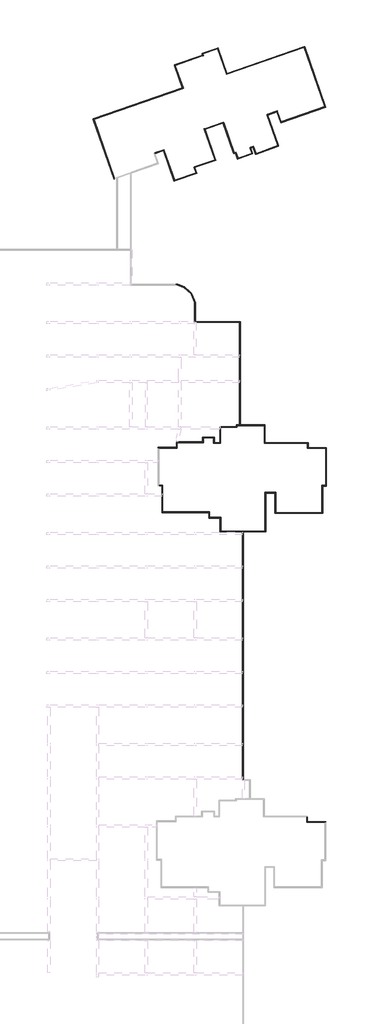
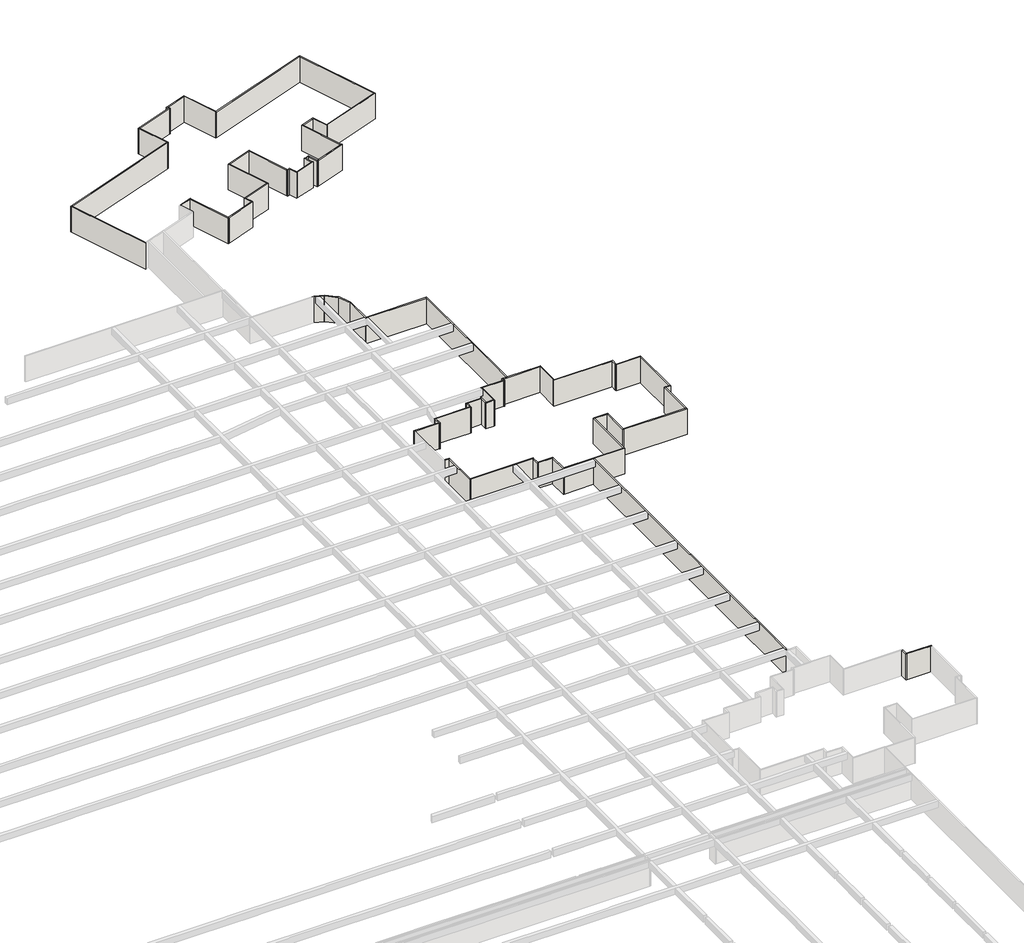
# One storey, part 6 of 14: 66 walls.
"""IFC4 building model written with IfcOpenShell, lengths in millimetres."""

from ifc_helpers import new_model, si_unit, origin, origin_with_axes, place, context, project, spatial, polyline, outline, extrude, faceted_brep, element, save

model = new_model("IFC4")

# Units and contexts
model_context = context("Model", 3, world=origin())
ifc_project = project(units=[si_unit("LENGTHUNIT", "METRE", prefix="MILLI")], contexts=[model_context])

# Site, building, storey
site = spatial("IfcSite", under=ifc_project)
building = spatial("IfcBuilding", under=site)
storey = spatial("IfcBuildingStorey", under=building, Name="户型图", Elevation=0.0)

# Walls
placement = place(None, origin())
element("IfcWall", 1, ObjectType="所有墙体", at=placement, inside=storey, context=model_context, shape_type="Brep", body=[
    faceted_brep([(-487731.9156201, -109117.5126628, 0.0), (-487731.9156201, -110017.5126628, 0.0), (-487731.9156201, -110017.5126628, 3300.0), (-487731.9156201, -109117.5126628, 3300.0), (-487611.9156201, -109117.5126628, 0.0), (-487611.9156201, -109117.5126628, 3300.0), (-487611.9156201, -109897.5126628, 3300.0), (-487611.9156201, -110017.5126628, 3300.0), (-487611.9156201, -110017.5126628, 0.0), (-487611.9156201, -109897.5126628, 0.0)], [[[0, 1, 2, 3]], [[4, 5, 6, 7, 8, 9]], [[1, 0, 4, 9, 8]], [[3, 2, 7, 6, 5]], [[0, 3, 5, 4]], [[2, 1, 8, 7]]]),
])
element("IfcWall", 2, ObjectType="所有墙体", at=placement, inside=storey, context=model_context, shape_type="Brep", body=[
    faceted_brep([(-487611.9156201, -110017.5126628, 0.0), (-484731.9156201, -110017.5126628, 0.0), (-484611.9156201, -110017.5126628, 0.0), (-484611.9156201, -110017.5126628, 3300.0), (-484731.9156201, -110017.5126628, 3300.0), (-487611.9156201, -110017.5126628, 3300.0), (-487611.9156201, -109897.5126628, 0.0), (-487611.9156201, -109897.5126628, 3300.0), (-484611.9156201, -109897.5126628, 3300.0), (-484611.9156201, -109897.5126628, 0.0)], [[[0, 1, 2, 3, 4, 5]], [[6, 7, 8, 9]], [[2, 1, 0, 6, 9]], [[5, 4, 3, 8, 7]], [[0, 5, 7, 6]], [[3, 2, 9, 8]]]),
])
element("IfcWall", 3, ObjectType="所有墙体", at=placement, inside=storey, context=model_context, shape_type="SweptSolid", body=[
    extrude(outline(polyline([(-498157.6529954, -62419.4327531), (-498157.6529954, -103033.8197785), (-498277.6529954, -103033.8197785), (-498277.6529954, -62419.4327531), (-498157.6529954, -62419.4327531)])), origin_with_axes(), (0.0, 0.0, 1.0), 3300.0),
])
element("IfcWall", 4, ObjectType="所有墙体", at=placement, inside=storey, context=model_context, shape_type="Brep", body=[
    faceted_brep([(-501839.5424455, -62419.4327531, 0.0), (-498277.6529954, -62419.4327531, 0.0), (-498157.6529954, -62419.4327531, 0.0), (-494448.2280208, -62419.4327531, 0.0), (-494448.2280208, -62419.4327531, 3300.0), (-498157.6529954, -62419.4327531, 3300.0), (-498277.6529954, -62419.4327531, 3300.0), (-501839.5424455, -62419.4327531, 3300.0), (-501839.5424455, -62299.4327531, 0.0), (-501839.5424455, -62299.4327531, 3300.0), (-494568.2280208, -62299.4327531, 3300.0), (-494448.2280208, -62299.4327531, 3300.0), (-494448.2280208, -62299.4327531, 0.0), (-494568.2280208, -62299.4327531, 0.0)], [[[0, 1, 2, 3, 4, 5, 6, 7]], [[8, 9, 10, 11, 12, 13]], [[3, 2, 1, 0, 8, 13, 12]], [[7, 6, 5, 4, 11, 10, 9]], [[4, 3, 12, 11]], [[0, 7, 9, 8]]]),
])
element("IfcWall", 5, ObjectType="所有墙体", at=placement, inside=storey, context=model_context, shape_type="Brep", body=[
    faceted_brep([(-494448.2280208, -62299.4327531, 0.0), (-494448.2280208, -56065.482039, 0.0), (-494448.2280208, -55945.482039, 0.0), (-494448.2280208, -55945.482039, 3300.0), (-494448.2280208, -56065.482039, 3300.0), (-494448.2280208, -62299.4327531, 3300.0), (-494568.2280208, -62299.4327531, 0.0), (-494568.2280208, -62299.4327531, 3300.0), (-494568.2280208, -55945.482039, 3300.0), (-494568.2280208, -55945.482039, 0.0)], [[[0, 1, 2, 3, 4, 5]], [[6, 7, 8, 9]], [[2, 1, 0, 6, 9]], [[5, 4, 3, 8, 7]], [[0, 5, 7, 6]], [[3, 2, 9, 8]]]),
])
element("IfcWall", 6, ObjectType="所有墙体", at=placement, inside=storey, context=model_context, shape_type="Brep", body=[
    faceted_brep([(-494448.2280208, -56065.482039, 0.0), (-492943.6459925, -56065.482039, 0.0), (-492823.6459925, -56065.482039, 0.0), (-492823.6459925, -56065.482039, 3300.0), (-492943.6459925, -56065.482039, 3300.0), (-494448.2280208, -56065.482039, 3300.0), (-494448.2280208, -55945.482039, 0.0), (-494448.2280208, -55945.482039, 3300.0), (-492823.6459925, -55945.482039, 3300.0), (-492823.6459925, -55945.482039, 0.0)], [[[0, 1, 2, 3, 4, 5]], [[6, 7, 8, 9]], [[2, 1, 0, 6, 9]], [[5, 4, 3, 8, 7]], [[0, 5, 7, 6]], [[3, 2, 9, 8]]]),
])
element("IfcWall", 7, ObjectType="所有墙体", at=placement, inside=storey, context=model_context, shape_type="Brep", body=[
    faceted_brep([(-492943.6459925, -56065.482039, 0.0), (-492943.6459925, -59371.7887885, 0.0), (-492943.6459925, -59371.7887885, 3300.0), (-492943.6459925, -56065.482039, 3300.0), (-492823.6459925, -56065.482039, 0.0), (-492823.6459925, -56065.482039, 3300.0), (-492823.6459925, -59251.7887885, 3300.0), (-492823.6459925, -59371.7887885, 3300.0), (-492823.6459925, -59371.7887885, 0.0), (-492823.6459925, -59251.7887885, 0.0)], [[[0, 1, 2, 3]], [[4, 5, 6, 7, 8, 9]], [[1, 0, 4, 9, 8]], [[3, 2, 7, 6, 5]], [[0, 3, 5, 4]], [[2, 1, 8, 7]]]),
])
element("IfcWall", 8, ObjectType="所有墙体", at=placement, inside=storey, context=model_context, shape_type="Brep", body=[
    faceted_brep([(-492823.6459925, -59371.7887885, 0.0), (-485136.3735207, -59371.7887885, 0.0), (-485136.3735207, -59371.7887885, 3300.0), (-492823.6459925, -59371.7887885, 3300.0), (-492823.6459925, -59251.7887885, 0.0), (-492823.6459925, -59251.7887885, 3300.0), (-485256.3735207, -59251.7887885, 3300.0), (-485136.3735207, -59251.7887885, 3300.0), (-485136.3735207, -59251.7887885, 0.0), (-485256.3735207, -59251.7887885, 0.0)], [[[0, 1, 2, 3]], [[4, 5, 6, 7, 8, 9]], [[1, 0, 4, 9, 8]], [[3, 2, 7, 6, 5]], [[0, 3, 5, 4]], [[2, 1, 8, 7]]]),
])
element("IfcWall", 9, ObjectType="所有墙体", at=placement, inside=storey, context=model_context, shape_type="Brep", body=[
    faceted_brep([(-485136.3735207, -59251.7887885, 0.0), (-485136.3735207, -54901.4809263, 0.0), (-485136.3735207, -54781.4809263, 0.0), (-485136.3735207, -54781.4809263, 3300.0), (-485136.3735207, -54901.4809263, 3300.0), (-485136.3735207, -59251.7887885, 3300.0), (-485256.3735207, -59251.7887885, 0.0), (-485256.3735207, -59251.7887885, 3300.0), (-485256.3735207, -54781.4809263, 3300.0), (-485256.3735207, -54781.4809263, 0.0)], [[[0, 1, 2, 3, 4, 5]], [[6, 7, 8, 9]], [[2, 1, 0, 6, 9]], [[5, 4, 3, 8, 7]], [[0, 5, 7, 6]], [[3, 2, 9, 8]]]),
])
element("IfcWall", 10, ObjectType="所有墙体", at=placement, inside=storey, context=model_context, shape_type="Brep", body=[
    faceted_brep([(-485136.3735207, -54901.4809263, 0.0), (-484519.0828774, -54901.4809263, 0.0), (-484519.0828774, -54901.4809263, 3300.0), (-485136.3735207, -54901.4809263, 3300.0), (-485136.3735207, -54781.4809263, 0.0), (-485136.3735207, -54781.4809263, 3300.0), (-484639.0828774, -54781.4809263, 3300.0), (-484519.0828774, -54781.4809263, 3300.0), (-484519.0828774, -54781.4809263, 0.0), (-484639.0828774, -54781.4809263, 0.0)], [[[0, 1, 2, 3]], [[4, 5, 6, 7, 8, 9]], [[1, 0, 4, 9, 8]], [[3, 2, 7, 6, 5]], [[0, 3, 5, 4]], [[2, 1, 8, 7]]]),
])
element("IfcWall", 11, ObjectType="所有墙体", at=placement, inside=storey, context=model_context, shape_type="Brep", body=[
    faceted_brep([(-484519.0828774, -54781.4809263, 0.0), (-484519.0828774, -48583.8215635, 0.0), (-484519.0828774, -48583.8215635, 3300.0), (-484519.0828774, -54781.4809263, 3300.0), (-484639.0828774, -54781.4809263, 0.0), (-484639.0828774, -54781.4809263, 3300.0), (-484639.0828774, -48703.8215635, 3300.0), (-484639.0828774, -48583.8215635, 3300.0), (-484639.0828774, -48583.8215635, 0.0), (-484639.0828774, -48703.8215635, 0.0)], [[[0, 1, 2, 3]], [[4, 5, 6, 7, 8, 9]], [[1, 0, 4, 9, 8]], [[3, 2, 7, 6, 5]], [[0, 3, 5, 4]], [[2, 1, 8, 7]]]),
])
element("IfcWall", 12, ObjectType="所有墙体", at=placement, inside=storey, context=model_context, shape_type="Brep", body=[
    faceted_brep([(-484639.0828774, -48583.8215635, 0.0), (-487495.1396851, -48583.8215635, 0.0), (-487615.1396851, -48583.8215635, 0.0), (-487615.1396851, -48583.8215635, 3300.0), (-487495.1396851, -48583.8215635, 3300.0), (-484639.0828774, -48583.8215635, 3300.0), (-484639.0828774, -48703.8215635, 0.0), (-484639.0828774, -48703.8215635, 3300.0), (-487615.1396851, -48703.8215635, 3300.0), (-487615.1396851, -48703.8215635, 0.0)], [[[0, 1, 2, 3, 4, 5]], [[6, 7, 8, 9]], [[2, 1, 0, 6, 9]], [[5, 4, 3, 8, 7]], [[0, 5, 7, 6]], [[3, 2, 9, 8]]]),
])
element("IfcWall", 13, ObjectType="所有墙体", at=placement, inside=storey, context=model_context, shape_type="Brep", body=[
    faceted_brep([(-487495.1396851, -48583.8215635, 0.0), (-487495.1396851, -47772.3075196, 0.0), (-487495.1396851, -47772.3075196, 3300.0), (-487495.1396851, -48583.8215635, 3300.0), (-487615.1396851, -48583.8215635, 0.0), (-487615.1396851, -48583.8215635, 3300.0), (-487615.1396851, -47892.3075196, 3300.0), (-487615.1396851, -47772.3075196, 3300.0), (-487615.1396851, -47772.3075196, 0.0), (-487615.1396851, -47892.3075196, 0.0)], [[[0, 1, 2, 3]], [[4, 5, 6, 7, 8, 9]], [[1, 0, 4, 9, 8]], [[3, 2, 7, 6, 5]], [[0, 3, 5, 4]], [[2, 1, 8, 7]]]),
])
element("IfcWall", 14, ObjectType="所有墙体", at=placement, inside=storey, context=model_context, shape_type="Brep", body=[
    faceted_brep([(-487615.1396851, -47772.3075196, 0.0), (-494595.1396851, -47772.3075196, 0.0), (-494715.1396851, -47772.3075196, 0.0), (-494715.1396851, -47772.3075196, 3300.0), (-494595.1396851, -47772.3075196, 3300.0), (-487615.1396851, -47772.3075196, 3300.0), (-487615.1396851, -47892.3075196, 0.0), (-487615.1396851, -47892.3075196, 3300.0), (-494715.1396851, -47892.3075196, 3300.0), (-494715.1396851, -47892.3075196, 0.0)], [[[0, 1, 2, 3, 4, 5]], [[6, 7, 8, 9]], [[2, 1, 0, 6, 9]], [[5, 4, 3, 8, 7]], [[0, 5, 7, 6]], [[3, 2, 9, 8]]]),
])
element("IfcWall", 15, ObjectType="所有墙体", at=placement, inside=storey, context=model_context, shape_type="Brep", body=[
    faceted_brep([(-494595.1396851, -47772.3075196, 0.0), (-494595.1396851, -44872.3075196, 0.0), (-494595.1396851, -44872.3075196, 3300.0), (-494595.1396851, -47772.3075196, 3300.0), (-494715.1396851, -47772.3075196, 0.0), (-494715.1396851, -47772.3075196, 3300.0), (-494715.1396851, -44992.3075196, 3300.0), (-494715.1396851, -44872.3075196, 3300.0), (-494715.1396851, -44872.3075196, 0.0), (-494715.1396851, -44992.3075196, 0.0)], [[[0, 1, 2, 3]], [[4, 5, 6, 7, 8, 9]], [[1, 0, 4, 9, 8]], [[3, 2, 7, 6, 5]], [[0, 3, 5, 4]], [[2, 1, 8, 7]]]),
])
element("IfcWall", 16, ObjectType="所有墙体", at=placement, inside=storey, context=model_context, shape_type="Brep", body=[
    faceted_brep([(-494715.1396851, -44872.3075196, 0.0), (-498635.1396851, -44872.3075196, 0.0), (-498755.1396851, -44872.3075196, 0.0), (-499195.1396851, -44872.3075196, 0.0), (-499195.1396851, -44872.3075196, 3300.0), (-498755.1396851, -44872.3075196, 3300.0), (-498635.1396851, -44872.3075196, 3300.0), (-494715.1396851, -44872.3075196, 3300.0), (-494715.1396851, -44992.3075196, 0.0), (-494715.1396851, -44992.3075196, 3300.0), (-499195.1396851, -44992.3075196, 3300.0), (-499195.1396851, -44992.3075196, 0.0)], [[[0, 1, 2, 3, 4, 5, 6, 7]], [[8, 9, 10, 11]], [[3, 2, 1, 0, 8, 11]], [[7, 6, 5, 4, 10, 9]], [[0, 7, 9, 8]], [[4, 3, 11, 10]]]),
])
element("IfcWall", 17, ObjectType="所有墙体", at=placement, inside=storey, context=model_context, shape_type="Brep", body=[
    faceted_brep([(-499315.1396851, -44872.3075196, 0.0), (-499315.1396851, -45172.3075196, 0.0), (-499315.1396851, -45292.3075196, 0.0), (-499315.1396851, -45292.3075196, 3300.0), (-499315.1396851, -45172.3075196, 3300.0), (-499315.1396851, -44872.3075196, 3300.0), (-499195.1396851, -44872.3075196, 0.0), (-499195.1396851, -44872.3075196, 3300.0), (-499195.1396851, -44992.3075196, 3300.0), (-499195.1396851, -45292.3075196, 3300.0), (-499195.1396851, -45292.3075196, 0.0), (-499195.1396851, -44992.3075196, 0.0)], [[[0, 1, 2, 3, 4, 5]], [[6, 7, 8, 9, 10, 11]], [[2, 1, 0, 6, 11, 10]], [[5, 4, 3, 9, 8, 7]], [[0, 5, 7, 6]], [[3, 2, 10, 9]]]),
])
element("IfcWall", 18, ObjectType="所有墙体", at=placement, inside=storey, context=model_context, shape_type="Brep", body=[
    faceted_brep([(-499315.1396851, -45172.3075196, 0.0), (-502015.1396851, -45172.3075196, 0.0), (-502015.1396851, -45172.3075196, 2500.0), (-502015.1396851, -45172.3075196, 3300.0), (-501895.1396851, -45172.3075196, 3300.0), (-499315.1396851, -45172.3075196, 3300.0), (-499315.1396851, -45292.3075196, 0.0), (-499315.1396851, -45292.3075196, 3300.0), (-501895.1396851, -45292.3075196, 3300.0), (-502015.1396851, -45292.3075196, 3300.0), (-502015.1396851, -45292.3075196, 0.0), (-501895.1396851, -45292.3075196, 0.0)], [[[0, 1, 2, 3, 4, 5]], [[6, 7, 8, 9, 10, 11]], [[1, 0, 6, 11, 10]], [[5, 4, 3, 9, 8, 7]], [[0, 5, 7, 6]], [[3, 2, 1, 10, 9]]]),
])
element("IfcWall", 19, ObjectType="所有墙体", at=placement, inside=storey, context=model_context, shape_type="Brep", body=[
    faceted_brep([(-502015.1396851, -45292.3075196, 0.0), (-502015.1396851, -47772.3075196, 0.0), (-502015.1396851, -47892.3075196, 0.0), (-502015.1396851, -47892.3075196, 3300.0), (-502015.1396851, -47772.3075196, 3300.0), (-502015.1396851, -45292.3075196, 3300.0), (-501895.1396851, -45292.3075196, 0.0), (-501895.1396851, -45292.3075196, 3300.0), (-501895.1396851, -47892.3075196, 3300.0), (-501895.1396851, -47892.3075196, 0.0)], [[[0, 1, 2, 3, 4, 5]], [[6, 7, 8, 9]], [[2, 1, 0, 6, 9]], [[5, 4, 3, 8, 7]], [[0, 5, 7, 6]], [[3, 2, 9, 8]]]),
])
element("IfcWall", 20, ObjectType="所有墙体", at=placement, inside=storey, context=model_context, shape_type="Brep", body=[
    faceted_brep([(-502015.1396851, -47772.3075196, 0.0), (-502895.1396851, -47772.3075196, 0.0), (-503015.1396851, -47772.3075196, 0.0), (-503015.1396851, -47772.3075196, 3300.0), (-502895.1396851, -47772.3075196, 3300.0), (-502015.1396851, -47772.3075196, 3300.0), (-502015.1396851, -47892.3075196, 0.0), (-502015.1396851, -47892.3075196, 3300.0), (-503015.1396851, -47892.3075196, 3300.0), (-503015.1396851, -47892.3075196, 0.0)], [[[0, 1, 2, 3, 4, 5]], [[6, 7, 8, 9]], [[2, 1, 0, 6, 9]], [[5, 4, 3, 8, 7]], [[0, 5, 7, 6]], [[3, 2, 9, 8]]]),
])
element("IfcWall", 21, ObjectType="所有墙体", at=placement, inside=storey, context=model_context, shape_type="Brep", body=[
    faceted_brep([(-502895.1396851, -47772.3075196, 0.0), (-502895.1396851, -46872.3075196, 0.0), (-502895.1396851, -46872.3075196, 3300.0), (-502895.1396851, -47772.3075196, 3300.0), (-503015.1396851, -47772.3075196, 0.0), (-503015.1396851, -47772.3075196, 3300.0), (-503015.1396851, -46992.3075196, 3300.0), (-503015.1396851, -46872.3075196, 3300.0), (-503015.1396851, -46872.3075196, 0.0), (-503015.1396851, -46992.3075196, 0.0)], [[[0, 1, 2, 3]], [[4, 5, 6, 7, 8, 9]], [[1, 0, 4, 9, 8]], [[3, 2, 7, 6, 5]], [[0, 3, 5, 4]], [[2, 1, 8, 7]]]),
])
element("IfcWall", 22, ObjectType="所有墙体", at=placement, inside=storey, context=model_context, shape_type="Brep", body=[
    faceted_brep([(-503015.1396851, -46872.3075196, 0.0), (-504815.1396851, -46872.3075196, 0.0), (-504815.1396851, -46872.3075196, 3300.0), (-503015.1396851, -46872.3075196, 3300.0), (-503015.1396851, -46992.3075196, 0.0), (-503015.1396851, -46992.3075196, 3300.0), (-504695.1396851, -46992.3075196, 3300.0), (-504815.1396851, -46992.3075196, 3300.0), (-504815.1396851, -46992.3075196, 0.0), (-504695.1396851, -46992.3075196, 0.0)], [[[0, 1, 2, 3]], [[4, 5, 6, 7, 8, 9]], [[1, 0, 4, 9, 8]], [[3, 2, 7, 6, 5]], [[0, 3, 5, 4]], [[2, 1, 8, 7]]]),
])
element("IfcWall", 23, ObjectType="所有墙体", at=placement, inside=storey, context=model_context, shape_type="Brep", body=[
    faceted_brep([(-504815.1396851, -46992.3075196, 0.0), (-504815.1396851, -47655.7967618, 0.0), (-504815.1396851, -47775.7967618, 0.0), (-504815.1396851, -47775.7967618, 3300.0), (-504815.1396851, -47655.7967618, 3300.0), (-504815.1396851, -46992.3075196, 3300.0), (-504695.1396851, -46992.3075196, 0.0), (-504695.1396851, -46992.3075196, 3300.0), (-504695.1396851, -47775.7967618, 3300.0), (-504695.1396851, -47775.7967618, 0.0)], [[[0, 1, 2, 3, 4, 5]], [[6, 7, 8, 9]], [[2, 1, 0, 6, 9]], [[5, 4, 3, 8, 7]], [[0, 5, 7, 6]], [[3, 2, 9, 8]]]),
])
element("IfcWall", 24, ObjectType="所有墙体", at=placement, inside=storey, context=model_context, shape_type="Brep", body=[
    faceted_brep([(-504815.1396851, -47655.7967618, 0.0), (-509115.1396851, -47655.7967618, 0.0), (-509115.1396851, -47655.7967618, 3300.0), (-504815.1396851, -47655.7967618, 3300.0), (-504815.1396851, -47775.7967618, 0.0), (-504815.1396851, -47775.7967618, 3300.0), (-508995.1396851, -47775.7967618, 3300.0), (-509115.1396851, -47775.7967618, 3300.0), (-509115.1396851, -47775.7967618, 0.0), (-508995.1396851, -47775.7967618, 0.0)], [[[0, 1, 2, 3]], [[4, 5, 6, 7, 8, 9]], [[1, 0, 4, 9, 8]], [[3, 2, 7, 6, 5]], [[0, 3, 5, 4]], [[2, 1, 8, 7]]]),
])
element("IfcWall", 25, ObjectType="所有墙体", at=placement, inside=storey, context=model_context, shape_type="Brep", body=[
    faceted_brep([(-509115.1396851, -47775.7967618, 0.0), (-509115.1396851, -48542.2511208, 0.0), (-509115.1396851, -48662.2511208, 0.0), (-509115.1396851, -48662.2511208, 3300.0), (-509115.1396851, -48542.2511208, 3300.0), (-509115.1396851, -47775.7967618, 3300.0), (-508995.1396851, -47775.7967618, 0.0), (-508995.1396851, -47775.7967618, 3300.0), (-508995.1396851, -48662.2511208, 3300.0), (-508995.1396851, -48662.2511208, 0.0)], [[[0, 1, 2, 3, 4, 5]], [[6, 7, 8, 9]], [[2, 1, 0, 6, 9]], [[5, 4, 3, 8, 7]], [[0, 5, 7, 6]], [[3, 2, 9, 8]]]),
])
element("IfcWall", 26, ObjectType="所有墙体", at=placement, inside=storey, context=model_context, shape_type="Brep", body=[
    faceted_brep([(-509115.1396851, -48542.2511208, 0.0), (-512115.1621146, -48542.2511208, 0.0), (-512115.1621146, -48542.2511208, 3300.0), (-509115.1396851, -48542.2511208, 3300.0), (-509115.1396851, -48662.2511208, 0.0), (-509115.1396851, -48662.2511208, 3300.0), (-511995.1621146, -48662.2511208, 3300.0), (-512115.1621146, -48662.2511208, 3300.0), (-512115.1621146, -48662.2511208, 0.0), (-511995.1621146, -48662.2511208, 0.0)], [[[0, 1, 2, 3]], [[4, 5, 6, 7, 8, 9]], [[1, 0, 4, 9, 8]], [[3, 2, 7, 6, 5]], [[0, 3, 5, 4]], [[2, 1, 8, 7]]]),
])
element("IfcWall", 27, ObjectType="所有墙体", at=placement, inside=storey, context=model_context, shape_type="Brep", body=[
    faceted_brep([(-511995.1621146, -54862.2511208, 0.0), (-511515.1621146, -54862.2511208, 0.0), (-511395.1621146, -54862.2511208, 0.0), (-511395.1621146, -54862.2511208, 3300.0), (-511515.1621146, -54862.2511208, 3300.0), (-511995.1621146, -54862.2511208, 3300.0), (-511995.1621146, -54742.2511208, 0.0), (-511995.1621146, -54742.2511208, 3300.0), (-511395.1621146, -54742.2511208, 3300.0), (-511395.1621146, -54742.2511208, 0.0)], [[[0, 1, 2, 3, 4, 5]], [[6, 7, 8, 9]], [[2, 1, 0, 6, 9]], [[5, 4, 3, 8, 7]], [[0, 5, 7, 6]], [[3, 2, 9, 8]]]),
])
element("IfcWall", 28, ObjectType="所有墙体", at=placement, inside=storey, context=model_context, shape_type="Brep", body=[
    faceted_brep([(-511515.1621146, -54862.2511208, 0.0), (-511515.1621146, -59259.003002, 0.0), (-511515.1621146, -59259.003002, 3300.0), (-511515.1621146, -54862.2511208, 3300.0), (-511395.1621146, -54862.2511208, 0.0), (-511395.1621146, -54862.2511208, 3300.0), (-511395.1621146, -59139.003002, 3300.0), (-511395.1621146, -59259.003002, 3300.0), (-511395.1621146, -59259.003002, 0.0), (-511395.1621146, -59139.003002, 0.0)], [[[0, 1, 2, 3]], [[4, 5, 6, 7, 8, 9]], [[1, 0, 4, 9, 8]], [[3, 2, 7, 6, 5]], [[0, 3, 5, 4]], [[2, 1, 8, 7]]]),
])
element("IfcWall", 29, ObjectType="所有墙体", at=placement, inside=storey, context=model_context, shape_type="Brep", body=[
    faceted_brep([(-511395.1621146, -59259.003002, 0.0), (-503815.1621146, -59259.003002, 0.0), (-503695.1621146, -59259.003002, 0.0), (-503695.1621146, -59259.003002, 3300.0), (-503815.1621146, -59259.003002, 3300.0), (-511395.1621146, -59259.003002, 3300.0), (-511395.1621146, -59139.003002, 0.0), (-511395.1621146, -59139.003002, 3300.0), (-503695.1621146, -59139.003002, 3300.0), (-503695.1621146, -59139.003002, 0.0)], [[[0, 1, 2, 3, 4, 5]], [[6, 7, 8, 9]], [[2, 1, 0, 6, 9]], [[5, 4, 3, 8, 7]], [[0, 5, 7, 6]], [[3, 2, 9, 8]]]),
])
element("IfcWall", 30, ObjectType="所有墙体", at=placement, inside=storey, context=model_context, shape_type="Brep", body=[
    faceted_brep([(-503815.1621146, -59259.003002, 0.0), (-503815.1621146, -60159.003002, 0.0), (-503815.1621146, -60159.003002, 3300.0), (-503815.1621146, -59259.003002, 3300.0), (-503695.1621146, -59259.003002, 0.0), (-503695.1621146, -59259.003002, 3300.0), (-503695.1621146, -60039.003002, 3300.0), (-503695.1621146, -60159.003002, 3300.0), (-503695.1621146, -60159.003002, 0.0), (-503695.1621146, -60039.003002, 0.0)], [[[0, 1, 2, 3]], [[4, 5, 6, 7, 8, 9]], [[1, 0, 4, 9, 8]], [[3, 2, 7, 6, 5]], [[0, 3, 5, 4]], [[2, 1, 8, 7]]]),
])
element("IfcWall", 31, ObjectType="所有墙体", at=placement, inside=storey, context=model_context, shape_type="Brep", body=[
    faceted_brep([(-503695.1621146, -60159.003002, 0.0), (-501959.5424455, -60159.003002, 0.0), (-501839.5424455, -60159.003002, 0.0), (-501839.5424455, -60159.003002, 3300.0), (-501959.5424455, -60159.003002, 3300.0), (-503695.1621146, -60159.003002, 3300.0), (-503695.1621146, -60039.003002, 0.0), (-503695.1621146, -60039.003002, 3300.0), (-501839.5424455, -60039.003002, 3300.0), (-501839.5424455, -60039.003002, 0.0)], [[[0, 1, 2, 3, 4, 5]], [[6, 7, 8, 9]], [[2, 1, 0, 6, 9]], [[5, 4, 3, 8, 7]], [[0, 5, 7, 6]], [[3, 2, 9, 8]]]),
])
element("IfcWall", 32, ObjectType="所有墙体", at=placement, inside=storey, context=model_context, shape_type="Brep", body=[
    faceted_brep([(-501959.5424455, -60159.003002, 0.0), (-501959.5424455, -62419.4327531, 0.0), (-501959.5424455, -62419.4327531, 3300.0), (-501959.5424455, -60159.003002, 3300.0), (-501839.5424455, -60159.003002, 0.0), (-501839.5424455, -60159.003002, 3300.0), (-501839.5424455, -62299.4327531, 3300.0), (-501839.5424455, -62419.4327531, 3300.0), (-501839.5424455, -62419.4327531, 0.0), (-501839.5424455, -62299.4327531, 0.0)], [[[0, 1, 2, 3]], [[4, 5, 6, 7, 8, 9]], [[1, 0, 4, 9, 8]], [[3, 2, 7, 6, 5]], [[0, 3, 5, 4]], [[2, 1, 8, 7]]]),
])
element("IfcWall", 33, ObjectType="所有墙体", at=placement, inside=storey, context=model_context, shape_type="Brep", body=[
    faceted_brep([(-498635.1396851, -44872.3075196, 0.0), (-498635.1396851, -27939.4327531, 0.0), (-498635.1396851, -27939.4327531, 3300.0), (-498635.1396851, -44872.3075196, 3300.0), (-498755.1396851, -44872.3075196, 0.0), (-498755.1396851, -44872.3075196, 3300.0), (-498755.1396851, -28059.4327531, 3300.0), (-498755.1396851, -27939.4327531, 3300.0), (-498755.1396851, -27939.4327531, 0.0), (-498755.1396851, -28059.4327531, 0.0)], [[[0, 1, 2, 3]], [[4, 5, 6, 7, 8, 9]], [[1, 0, 4, 9, 8]], [[3, 2, 7, 6, 5]], [[0, 3, 5, 4]], [[2, 1, 8, 7]]]),
])
element("IfcWall", 34, ObjectType="所有墙体", at=placement, inside=storey, context=model_context, shape_type="Brep", body=[
    faceted_brep([(-498755.1396851, -27939.4327531, 0.0), (-506035.1396851, -27939.4327531, 0.0), (-506155.1396851, -27939.4327531, 0.0), (-506155.1396851, -27939.4327531, 3300.0), (-506035.1396851, -27939.4327531, 3300.0), (-498755.1396851, -27939.4327531, 3300.0), (-498755.1396851, -28059.4327531, 0.0), (-498755.1396851, -28059.4327531, 3300.0), (-506067.6529954, -28059.4327531, 3300.0), (-506155.1396851, -28059.4327531, 3300.0), (-506155.1396851, -28059.4327531, 2500.0), (-506155.1396851, -28059.4327531, 0.0)], [[[0, 1, 2, 3, 4, 5]], [[6, 7, 8, 9, 10, 11]], [[2, 1, 0, 6, 11]], [[5, 4, 3, 9, 8, 7]], [[0, 5, 7, 6]], [[3, 2, 11, 10, 9]]]),
])
element("IfcWall", 35, ObjectType="所有墙体", at=placement, inside=storey, context=model_context, shape_type="Brep", body=[
    faceted_brep([(-506035.1396851, -27939.4327531, 0.0), (-506035.1396851, -24747.7021405, 0.0), (-506035.1396851, -24747.7021405, 3300.0), (-506035.1396851, -27939.4327531, 3300.0), (-506155.1396851, -27939.4327531, 0.0), (-506155.1396851, -27939.4327531, 3300.0), (-506155.1396851, -27859.4327531, 3300.0), (-506155.1396851, -24771.1633658, 3300.0), (-506155.1396851, -24452.5434105, 3300.0), (-506155.1396851, -24452.5434105, 0.0), (-506155.1396851, -24771.1633658, 0.0)], [[[0, 1, 2, 3]], [[4, 5, 6, 7, 8, 9, 10]], [[1, 0, 4, 10, 9]], [[3, 2, 8, 7, 6, 5]], [[0, 3, 5, 4]], [[2, 1, 9, 8]]]),
])
element("IfcWall", 36, ObjectType="所有墙体", at=placement, inside=storey, context=model_context, shape_type="Brep", body=[
    faceted_brep([(-506155.1396851, -24452.5434105, 0.0), (-506634.5565644, -23273.3427667, 0.0), (-506634.5565644, -23273.3427667, 3300.0), (-506155.1396851, -24452.5434105, 3300.0), (-506155.1396851, -24771.1633658, 0.0), (-506155.1396851, -24771.1633658, 3300.0), (-506734.7494264, -23345.5227396, 3300.0), (-506833.3243097, -23103.0624283, 3300.0), (-506833.3243097, -23103.0624283, 0.0), (-506734.7494264, -23345.5227396, 0.0)], [[[0, 1, 2, 3]], [[4, 5, 6, 7, 8, 9]], [[1, 0, 4, 9, 8]], [[3, 2, 7, 6, 5]], [[0, 3, 5, 4]], [[2, 1, 8, 7]]]),
])
element("IfcWall", 37, ObjectType="所有墙体", at=placement, inside=storey, context=model_context, shape_type="SweptSolid", body=[
    extrude(outline(polyline([(-507820.7587047, -22257.147198), (-506833.3243097, -23103.0624283), (-506734.7494264, -23345.5227396), (-507883.1414859, -22361.7183083), (-507820.7587047, -22257.147198)])), origin_with_axes(), (0.0, 0.0, 1.0), 3300.0),
])
element("IfcWall", 38, ObjectType="所有墙体", at=placement, inside=storey, context=model_context, shape_type="Brep", body=[
    faceted_brep([(-507820.7587047, -22257.147198, 0.0), (-508906.5049791, -21839.2569935, 0.0), (-508906.5049791, -21839.2569935, 3300.0), (-507820.7587047, -22257.147198, 3300.0), (-507883.1414859, -22361.7183083, 0.0), (-507883.1414859, -22361.7183083, 3300.0), (-508928.8010117, -21959.2569935, 3300.0), (-509240.5804015, -21839.2569935, 3300.0), (-509240.5804015, -21839.2569935, 0.0), (-508928.8010117, -21959.2569935, 0.0)], [[[0, 1, 2, 3]], [[4, 5, 6, 7, 8, 9]], [[1, 0, 4, 9, 8]], [[3, 2, 7, 6, 5]], [[0, 3, 5, 4]], [[2, 1, 8, 7]]]),
])
element("IfcWall", 39, ObjectType="所有墙体", at=placement, inside=storey, context=model_context, shape_type="Brep", body=[
    faceted_brep([(-512675.4931907, -384.9532556, 0.0), (-511246.2354826, 111.3129454, 0.0), (-511132.8745486, 150.6740766, 0.0), (-511132.8745486, 150.6740766, 3300.0), (-511246.2354826, 111.3129454, 3300.0), (-512675.4931907, -384.9532556, 3300.0), (-512714.8543218, -271.5923217, 0.0), (-512714.8543218, -271.5923217, 3300.0), (-511172.2356797, 264.0350106, 3300.0), (-511172.2356797, 264.0350106, 0.0)], [[[0, 1, 2, 3, 4, 5]], [[6, 7, 8, 9]], [[2, 1, 0, 6, 9]], [[5, 4, 3, 8, 7]], [[0, 5, 7, 6]], [[3, 2, 9, 8]]]),
])
element("IfcWall", 40, ObjectType="所有墙体", at=placement, inside=storey, context=model_context, shape_type="Brep", body=[
    faceted_brep([(-511246.2354826, 111.3129454, 0.0), (-509502.0327403, -4912.0297855, 0.0), (-509502.0327403, -4912.0297855, 3300.0), (-511246.2354826, 111.3129454, 3300.0), (-511132.8745486, 150.6740766, 0.0), (-511132.8745486, 150.6740766, 3300.0), (-509428.0329375, -4759.3077204, 3300.0), (-509388.6718063, -4872.6686544, 3300.0), (-509388.6718063, -4872.6686544, 0.0), (-509428.0329375, -4759.3077204, 0.0)], [[[0, 1, 2, 3]], [[4, 5, 6, 7, 8, 9]], [[1, 0, 4, 9, 8]], [[3, 2, 7, 6, 5]], [[0, 3, 5, 4]], [[2, 1, 8, 7]]]),
])
element("IfcWall", 41, ObjectType="所有墙体", at=placement, inside=storey, context=model_context, shape_type="Brep", body=[
    faceted_brep([(-509388.6718063, -4872.6686544, 0.0), (-505756.5673718, -3611.5310307, 0.0), (-505756.5673718, -3611.5310307, 3300.0), (-509388.6718063, -4872.6686544, 3300.0), (-509428.0329375, -4759.3077204, 0.0), (-509428.0329375, -4759.3077204, 3300.0), (-505910.7131052, -3538.0255532, 3300.0), (-505797.3433424, -3498.6613566, 3300.0), (-505797.3433424, -3498.6613566, 0.0), (-505910.7131052, -3538.0255532, 0.0)], [[[0, 1, 2, 3]], [[4, 5, 6, 7, 8, 9]], [[1, 0, 4, 9, 8]], [[3, 2, 7, 6, 5]], [[0, 3, 5, 4]], [[2, 1, 8, 7]]]),
])
element("IfcWall", 42, ObjectType="所有墙体", at=placement, inside=storey, context=model_context, shape_type="Brep", body=[
    faceted_brep([(-505797.3433424, -3498.6613566, 0.0), (-506096.3406643, -2671.0236624, 0.0), (-506137.1166349, -2558.1539883, 0.0), (-506137.1166349, -2558.1539883, 3300.0), (-506096.3406643, -2671.0236624, 3300.0), (-505797.3433424, -3498.6613566, 3300.0), (-505910.7131052, -3538.0255532, 0.0), (-505910.7131052, -3538.0255532, 3300.0), (-506250.4863977, -2597.518185, 3300.0), (-506250.4863977, -2597.518185, 0.0)], [[[0, 1, 2, 3, 4, 5]], [[6, 7, 8, 9]], [[2, 1, 0, 6, 9]], [[5, 4, 3, 8, 7]], [[0, 5, 7, 6]], [[3, 2, 9, 8]]]),
])
element("IfcWall", 43, ObjectType="所有墙体", at=placement, inside=storey, context=model_context, shape_type="Brep", body=[
    faceted_brep([(-506096.3406643, -2671.0236624, 0.0), (-502674.2711366, -1482.814262, 0.0), (-502674.2711366, -1482.814262, 3300.0), (-506096.3406643, -2671.0236624, 3300.0), (-506137.1166349, -2558.1539883, 0.0), (-506137.1166349, -2558.1539883, 3300.0), (-502826.9932017, -1408.8144591, 3300.0), (-502713.6322677, -1369.453328, 3300.0), (-502713.6322677, -1369.453328, 0.0), (-502826.9932017, -1408.8144591, 0.0)], [[[0, 1, 2, 3]], [[4, 5, 6, 7, 8, 9]], [[1, 0, 4, 9, 8]], [[3, 2, 7, 6, 5]], [[0, 3, 5, 4]], [[2, 1, 8, 7]]]),
])
element("IfcWall", 44, ObjectType="所有墙体", at=placement, inside=storey, context=model_context, shape_type="Brep", body=[
    faceted_brep([(-502713.6322677, -1369.453328, 0.0), (-504436.2457457, 3591.7118413, 0.0), (-504475.6068769, 3705.0727753, 0.0), (-504475.6068769, 3705.0727753, 3300.0), (-504436.2457457, 3591.7118413, 3300.0), (-502713.6322677, -1369.453328, 3300.0), (-502826.9932017, -1408.8144591, 0.0), (-502826.9932017, -1408.8144591, 3300.0), (-504588.9678109, 3665.7116442, 3300.0), (-504588.9678109, 3665.7116442, 0.0)], [[[0, 1, 2, 3, 4, 5]], [[6, 7, 8, 9]], [[2, 1, 0, 6, 9]], [[5, 4, 3, 8, 7]], [[0, 5, 7, 6]], [[3, 2, 9, 8]]]),
])
element("IfcWall", 45, ObjectType="所有墙体", at=placement, inside=storey, context=model_context, shape_type="Brep", body=[
    faceted_brep([(-504436.2457457, 3591.7118413, 0.0), (-501472.8947804, 4620.6451944, 0.0), (-501359.5338464, 4660.0063256, 0.0), (-501359.5338464, 4660.0063256, 3300.0), (-501472.8947804, 4620.6451944, 3300.0), (-504436.2457457, 3591.7118413, 3300.0), (-504475.6068769, 3705.0727753, 0.0), (-504475.6068769, 3705.0727753, 3300.0), (-501398.8949775, 4773.3672596, 3300.0), (-501398.8949775, 4773.3672596, 0.0)], [[[0, 1, 2, 3, 4, 5]], [[6, 7, 8, 9]], [[2, 1, 0, 6, 9]], [[5, 4, 3, 8, 7]], [[0, 5, 7, 6]], [[3, 2, 9, 8]]]),
])
element("IfcWall", 46, ObjectType="所有墙体", at=placement, inside=storey, context=model_context, shape_type="SweptSolid", body=[
    extrude(outline(polyline([(-499750.0372052, -341.2229802), (-501472.8947804, 4620.6451944), (-501359.5338464, 4660.0063256), (-499637.1675311, -300.4470096), (-499750.0372052, -341.2229802)])), origin_with_axes(), (0.0, 0.0, 1.0), 3300.0),
])
element("IfcWall", 47, ObjectType="所有墙体", at=placement, inside=storey, context=model_context, shape_type="Brep", body=[
    faceted_brep([(-499710.6730085, -454.592743, 0.0), (-499428.520798, -352.6607553, 0.0), (-499315.6511239, -311.8847847, 0.0), (-499315.6511239, -311.8847847, 3300.0), (-499428.520798, -352.6607553, 3300.0), (-499710.6730085, -454.592743, 3300.0), (-499750.0372052, -341.2229802, 0.0), (-499750.0372052, -341.2229802, 3300.0), (-499637.1675311, -300.4470096, 3300.0), (-499355.0153206, -198.5150218, 3300.0), (-499355.0153206, -198.5150218, 0.0), (-499637.1675311, -300.4470096, 0.0)], [[[0, 1, 2, 3, 4, 5]], [[6, 7, 8, 9, 10, 11]], [[2, 1, 0, 6, 11, 10]], [[5, 4, 3, 9, 8, 7]], [[0, 5, 7, 6]], [[3, 2, 10, 9]]]),
])
element("IfcWall", 48, ObjectType="所有墙体", at=placement, inside=storey, context=model_context, shape_type="Brep", body=[
    faceted_brep([(-499428.520798, -352.6607553, 0.0), (-499099.5560248, -1300.0866263, 0.0), (-499099.5560248, -1300.0866263, 3300.0), (-499428.520798, -352.6607553, 3300.0), (-499315.6511239, -311.8847847, 0.0), (-499315.6511239, -311.8847847, 3300.0), (-499025.5562219, -1147.3645612, 3300.0), (-498986.1950908, -1260.7254952, 3300.0), (-498986.1950908, -1260.7254952, 0.0), (-499025.5562219, -1147.3645612, 0.0)], [[[0, 1, 2, 3]], [[4, 5, 6, 7, 8, 9]], [[1, 0, 4, 9, 8]], [[3, 2, 7, 6, 5]], [[0, 3, 5, 4]], [[2, 1, 8, 7]]]),
])
element("IfcWall", 49, ObjectType="所有墙体", at=placement, inside=storey, context=model_context, shape_type="Brep", body=[
    faceted_brep([(-498986.1950908, -1260.7254952, 0.0), (-496617.0428907, -438.1095628, 0.0), (-496617.0428907, -438.1095628, 3300.0), (-498986.1950908, -1260.7254952, 3300.0), (-499025.5562219, -1147.3645612, 0.0), (-499025.5562219, -1147.3645612, 3300.0), (-496769.7649558, -364.1097599, 3300.0), (-496656.4040218, -324.7486288, 3300.0), (-496656.4040218, -324.7486288, 0.0), (-496769.7649558, -364.1097599, 0.0)], [[[0, 1, 2, 3]], [[4, 5, 6, 7, 8, 9]], [[1, 0, 4, 9, 8]], [[3, 2, 7, 6, 5]], [[0, 3, 5, 4]], [[2, 1, 8, 7]]]),
])
element("IfcWall", 50, ObjectType="所有墙体", at=placement, inside=storey, context=model_context, shape_type="Brep", body=[
    faceted_brep([(-496656.4040218, -324.7486288, 0.0), (-496945.0267725, 506.4913192, 0.0), (-496984.3879036, 619.8522532, 0.0), (-496984.3879036, 619.8522532, 3300.0), (-496945.0267725, 506.4913192, 3300.0), (-496656.4040218, -324.7486288, 3300.0), (-496769.7649558, -364.1097599, 0.0), (-496769.7649558, -364.1097599, 3300.0), (-497097.7488376, 580.4911221, 3300.0), (-497097.7488376, 580.4911221, 0.0)], [[[0, 1, 2, 3, 4, 5]], [[6, 7, 8, 9]], [[2, 1, 0, 6, 9]], [[5, 4, 3, 8, 7]], [[0, 5, 7, 6]], [[3, 2, 9, 8]]]),
])
element("IfcWall", 51, ObjectType="所有墙体", at=placement, inside=storey, context=model_context, shape_type="Brep", body=[
    faceted_brep([(-496945.0267725, 506.4913192, 0.0), (-496552.4316225, 642.8080258, 0.0), (-496439.0706885, 682.1691569, 0.0), (-496439.0706885, 682.1691569, 3300.0), (-496552.4316225, 642.8080258, 3300.0), (-496945.0267725, 506.4913192, 3300.0), (-496984.3879036, 619.8522532, 0.0), (-496984.3879036, 619.8522532, 3300.0), (-496478.4318196, 795.5300909, 3300.0), (-496478.4318196, 795.5300909, 0.0)], [[[0, 1, 2, 3, 4, 5]], [[6, 7, 8, 9]], [[2, 1, 0, 6, 9]], [[5, 4, 3, 8, 7]], [[0, 5, 7, 6]], [[3, 2, 9, 8]]]),
])
element("IfcWall", 52, ObjectType="所有墙体", at=placement, inside=storey, context=model_context, shape_type="Brep", body=[
    faceted_brep([(-496552.4316225, 642.8080258, 0.0), (-496142.7167695, -537.1798727, 0.0), (-496142.7167695, -537.1798727, 3300.0), (-496552.4316225, 642.8080258, 3300.0), (-496439.0706885, 682.1691569, 0.0), (-496439.0706885, 682.1691569, 3300.0), (-496069.2112921, -383.0341393, 3300.0), (-496029.8470954, -496.4039022, 3300.0), (-496029.8470954, -496.4039022, 0.0), (-496069.2112921, -383.0341393, 0.0)], [[[0, 1, 2, 3]], [[4, 5, 6, 7, 8, 9]], [[1, 0, 4, 9, 8]], [[3, 2, 7, 6, 5]], [[0, 3, 5, 4]], [[2, 1, 8, 7]]]),
])
element("IfcWall", 53, ObjectType="所有墙体", at=placement, inside=storey, context=model_context, shape_type="Brep", body=[
    faceted_brep([(-496029.8470954, -496.4039022, 0.0), (-492361.8683593, 828.7119385, 0.0), (-492361.8683593, 828.7119385, 3300.0), (-496029.8470954, -496.4039022, 3300.0), (-496069.2112921, -383.0341393, 0.0), (-496069.2112921, -383.0341393, 3300.0), (-492514.10223, 901.3057308, 3300.0), (-492401.2325559, 942.0817013, 3300.0), (-492401.2325559, 942.0817013, 0.0), (-492514.10223, 901.3057308, 0.0)], [[[0, 1, 2, 3]], [[4, 5, 6, 7, 8, 9]], [[1, 0, 4, 9, 8]], [[3, 2, 7, 6, 5]], [[0, 3, 5, 4]], [[2, 1, 8, 7]]]),
])
element("IfcWall", 54, ObjectType="所有墙体", at=placement, inside=storey, context=model_context, shape_type="Brep", body=[
    faceted_brep([(-492401.2325559, 942.0817013, 0.0), (-494132.8751629, 5929.250963, 0.0), (-494172.236294, 6042.611897, 0.0), (-494172.236294, 6042.611897, 3300.0), (-494132.8751629, 5929.250963, 3300.0), (-492401.2325559, 942.0817013, 3300.0), (-492514.10223, 901.3057308, 0.0), (-492514.10223, 901.3057308, 3300.0), (-494285.597228, 6003.2507658, 3300.0), (-494285.597228, 6003.2507658, 0.0)], [[[0, 1, 2, 3, 4, 5]], [[6, 7, 8, 9]], [[2, 1, 0, 6, 9]], [[5, 4, 3, 8, 7]], [[0, 5, 7, 6]], [[3, 2, 9, 8]]]),
])
element("IfcWall", 55, ObjectType="所有墙体", at=placement, inside=storey, context=model_context, shape_type="Brep", body=[
    faceted_brep([(-494132.8751629, 5929.250963, 0.0), (-492640.289532, 6447.5058562, 0.0), (-492526.928598, 6486.8669873, 0.0), (-492526.928598, 6486.8669873, 3300.0), (-492640.289532, 6447.5058562, 3300.0), (-494132.8751629, 5929.250963, 3300.0), (-494172.236294, 6042.611897, 0.0), (-494172.236294, 6042.611897, 3300.0), (-492566.2897291, 6600.2279213, 3300.0), (-492566.2897291, 6600.2279213, 0.0)], [[[0, 1, 2, 3, 4, 5]], [[6, 7, 8, 9]], [[2, 1, 0, 6, 9]], [[5, 4, 3, 8, 7]], [[0, 5, 7, 6]], [[3, 2, 9, 8]]]),
])
element("IfcWall", 56, ObjectType="所有墙体", at=placement, inside=storey, context=model_context, shape_type="Brep", body=[
    faceted_brep([(-492640.289532, 6447.5058562, 0.0), (-492017.0716224, 4652.6244013, 0.0), (-492017.0716224, 4652.6244013, 3300.0), (-492640.289532, 6447.5058562, 3300.0), (-492526.928598, 6486.8669873, 0.0), (-492526.928598, 6486.8669873, 3300.0), (-491943.0718196, 4805.3464664, 3300.0), (-491903.7106884, 4691.9855324, 3300.0), (-491903.7106884, 4691.9855324, 0.0), (-491943.0718196, 4805.3464664, 0.0)], [[[0, 1, 2, 3]], [[4, 5, 6, 7, 8, 9]], [[1, 0, 4, 9, 8]], [[3, 2, 7, 6, 5]], [[0, 3, 5, 4]], [[2, 1, 8, 7]]]),
])
element("IfcWall", 57, ObjectType="所有墙体", at=placement, inside=storey, context=model_context, shape_type="Brep", body=[
    faceted_brep([(-491903.7106884, 4691.9855324, 0.0), (-484629.7174237, 7217.6581132, 0.0), (-484629.7174237, 7217.6581132, 3300.0), (-491903.7106884, 4691.9855324, 3300.0), (-491943.0718196, 4805.3464664, 0.0), (-491943.0718196, 4805.3464664, 3300.0), (-484782.4394889, 7291.657916, 3300.0), (-484669.0785549, 7331.0190472, 3300.0), (-484669.0785549, 7331.0190472, 0.0), (-484782.4394889, 7291.657916, 0.0)], [[[0, 1, 2, 3]], [[4, 5, 6, 7, 8, 9]], [[1, 0, 4, 9, 8]], [[3, 2, 7, 6, 5]], [[0, 3, 5, 4]], [[2, 1, 8, 7]]]),
])
element("IfcWall", 58, ObjectType="所有墙体", at=placement, inside=storey, context=model_context, shape_type="Brep", body=[
    faceted_brep([(-484669.0785549, 7331.0190472, 0.0), (-488080.3765861, 17155.6333267, 0.0), (-488080.3765861, 17155.6333267, 3300.0), (-484669.0785549, 7331.0190472, 3300.0), (-484782.4394889, 7291.657916, 0.0), (-484782.4394889, 7291.657916, 3300.0), (-488154.3763889, 17002.9112616, 3300.0), (-488193.7375201, 17116.2721956, 3300.0), (-488193.7375201, 17116.2721956, 0.0), (-488154.3763889, 17002.9112616, 0.0)], [[[0, 1, 2, 3]], [[4, 5, 6, 7, 8, 9]], [[1, 0, 4, 9, 8]], [[3, 2, 7, 6, 5]], [[0, 3, 5, 4]], [[2, 1, 8, 7]]]),
])
element("IfcWall", 59, ObjectType="所有墙体", at=placement, inside=storey, context=model_context, shape_type="Brep", body=[
    faceted_brep([(-488193.7375201, 17116.2721956, 0.0), (-500833.4816605, 12727.5060747, 0.0), (-500946.8425945, 12688.1449436, 0.0), (-500946.8425945, 12688.1449436, 3300.0), (-500833.4816605, 12727.5060747, 3300.0), (-488193.7375201, 17116.2721956, 3300.0), (-488154.3763889, 17002.9112616, 0.0), (-488154.3763889, 17002.9112616, 3300.0), (-500907.4814634, 12574.7840096, 3300.0), (-500907.4814634, 12574.7840096, 0.0)], [[[0, 1, 2, 3, 4, 5]], [[6, 7, 8, 9]], [[2, 1, 0, 6, 9]], [[5, 4, 3, 8, 7]], [[0, 5, 7, 6]], [[3, 2, 9, 8]]]),
])
element("IfcWall", 60, ObjectType="所有墙体", at=placement, inside=storey, context=model_context, shape_type="Brep", body=[
    faceted_brep([(-500833.4816605, 12727.5060747, 0.0), (-502294.5895999, 16935.5294706, 0.0), (-502294.5895999, 16935.5294706, 3300.0), (-500833.4816605, 12727.5060747, 3300.0), (-500946.8425945, 12688.1449436, 0.0), (-500946.8425945, 12688.1449436, 3300.0), (-502368.5894028, 16782.8074055, 3300.0), (-502407.9505339, 16896.1683395, 3300.0), (-502407.9505339, 16896.1683395, 0.0), (-502368.5894028, 16782.8074055, 0.0)], [[[0, 1, 2, 3]], [[4, 5, 6, 7, 8, 9]], [[1, 0, 4, 9, 8]], [[3, 2, 7, 6, 5]], [[0, 3, 5, 4]], [[2, 1, 8, 7]]]),
])
element("IfcWall", 61, ObjectType="所有墙体", at=placement, inside=storey, context=model_context, shape_type="SweptSolid", body=[
    extrude(outline(polyline([(-504845.2106148, 16049.9040202), (-502407.9505339, 16896.1683395), (-502368.5894028, 16782.8074055), (-504805.8494837, 15936.5430862), (-504845.2106148, 16049.9040202)])), origin_with_axes(), (0.0, 0.0, 1.0), 3300.0),
])
element("IfcWall", 62, ObjectType="所有墙体", at=placement, inside=storey, context=model_context, shape_type="Brep", body=[
    faceted_brep([(-504958.5715488, 16010.5428891, 0.0), (-504869.5148513, 15754.0576174, 0.0), (-504830.1537202, 15640.6966834, 0.0), (-504830.1537202, 15640.6966834, 3300.0), (-504869.5148513, 15754.0576174, 3300.0), (-504958.5715488, 16010.5428891, 3300.0), (-504845.2106148, 16049.9040202, 0.0), (-504845.2106148, 16049.9040202, 3300.0), (-504805.8494837, 15936.5430862, 3300.0), (-504716.7927862, 15680.0578145, 3300.0), (-504716.7927862, 15680.0578145, 0.0), (-504805.8494837, 15936.5430862, 0.0)], [[[0, 1, 2, 3, 4, 5]], [[6, 7, 8, 9, 10, 11]], [[2, 1, 0, 6, 11, 10]], [[5, 4, 3, 9, 8, 7]], [[0, 5, 7, 6]], [[3, 2, 10, 9]]]),
])
element("IfcWall", 63, ObjectType="所有墙体", at=placement, inside=storey, context=model_context, shape_type="Brep", body=[
    faceted_brep([(-504869.5148513, 15754.0576174, 0.0), (-509471.8402123, 14156.0403318, 0.0), (-509471.8402123, 14156.0403318, 3300.0), (-504869.5148513, 15754.0576174, 3300.0), (-504830.1537202, 15640.6966834, 0.0), (-504830.1537202, 15640.6966834, 3300.0), (-509319.1181472, 14082.040529, 3300.0), (-509432.4790812, 14042.6793978, 3300.0), (-509432.4790812, 14042.6793978, 0.0), (-509319.1181472, 14082.040529, 0.0)], [[[0, 1, 2, 3]], [[4, 5, 6, 7, 8, 9]], [[1, 0, 4, 9, 8]], [[3, 2, 7, 6, 5]], [[0, 3, 5, 4]], [[2, 1, 8, 7]]]),
])
element("IfcWall", 64, ObjectType="所有墙体", at=placement, inside=storey, context=model_context, shape_type="Brep", body=[
    faceted_brep([(-509432.4790812, 14042.6793978, 0.0), (-508159.802508, 10377.342532, 0.0), (-508120.4413769, 10263.981598, 0.0), (-508120.4413769, 10263.981598, 3300.0), (-508159.802508, 10377.342532, 3300.0), (-509432.4790812, 14042.6793978, 3300.0), (-509319.1181472, 14082.040529, 0.0), (-509319.1181472, 14082.040529, 3300.0), (-508007.0804429, 10303.3427291, 3300.0), (-508007.0804429, 10303.3427291, 0.0)], [[[0, 1, 2, 3, 4, 5]], [[6, 7, 8, 9]], [[2, 1, 0, 6, 9]], [[5, 4, 3, 8, 7]], [[0, 5, 7, 6]], [[3, 2, 9, 8]]]),
])
element("IfcWall", 65, ObjectType="所有墙体", at=placement, inside=storey, context=model_context, shape_type="Brep", body=[
    faceted_brep([(-508159.802508, 10377.342532, 0.0), (-522802.2564823, 5293.1964278, 0.0), (-522802.2564823, 5293.1964278, 3300.0), (-508159.802508, 10377.342532, 3300.0), (-508120.4413769, 10263.981598, 0.0), (-508120.4413769, 10263.981598, 3300.0), (-522649.5344172, 5219.1966249, 3300.0), (-522762.8953512, 5179.8354938, 3300.0), (-522762.8953512, 5179.8354938, 0.0), (-522649.5344172, 5219.1966249, 0.0)], [[[0, 1, 2, 3]], [[4, 5, 6, 7, 8, 9]], [[1, 0, 4, 9, 8]], [[3, 2, 7, 6, 5]], [[0, 3, 5, 4]], [[2, 1, 8, 7]]]),
])
element("IfcWall", 66, ObjectType="所有墙体", at=placement, inside=storey, context=model_context, shape_type="Brep", body=[
    faceted_brep([(-522762.8953512, 5179.8354938, 0.0), (-519378.854333, -4566.2779815, 0.0), (-519378.854333, -4566.2779815, 3300.0), (-522762.8953512, 5179.8354938, 3300.0), (-522649.5344172, 5219.1966249, 0.0), (-522649.5344172, 5219.1966249, 3300.0), (-519305.3488556, -4412.1322481, 3300.0), (-519265.9846589, -4525.5020109, 3300.0), (-519265.9846589, -4525.5020109, 0.0), (-519305.3488556, -4412.1322481, 0.0)], [[[0, 1, 2, 3]], [[4, 5, 6, 7, 8, 9]], [[1, 0, 4, 9, 8]], [[3, 2, 7, 6, 5]], [[0, 3, 5, 4]], [[2, 1, 8, 7]]]),
])

save(model, "model.ifc")

# Revit data of these elements
# Type "所有墙体"
#   Layers, outside or top first: 120 mm "默认" (function 1)
# Elements 1, 2, 3, 4, 5, 6, 7, 8, 9, 10, 11, 12, 13, 14, 15, 16, 17, 18, 19, 20, 21, 22, 23, 24, 25, 26, 27, 28, 29, 30, 31, 32, 33, 34, 35, 36, 37, 38, 39, 40, 41, 42, 43, 44, 45, 46, 47, 48, 49, 50, 51, 52, 53, 54, 55, 56, 57, 58, 59, 60, 61, 62, 63, 64, 65, 66 (IfcWall, "所有墙体")
#   Comments = ""
#   Top Offset = 0 mm
#   Base Offset = 0 mm
#   wall height = 3300 mm
#   Phase Created = 新构造
#   Base Constraint = 户型图
#   Top Constraint = 层高
#   Materials on its faces: "默认"
# Materials
#   "默认": class "其他", colour RGB 192 192 192, transparency 0, Cost = 0
